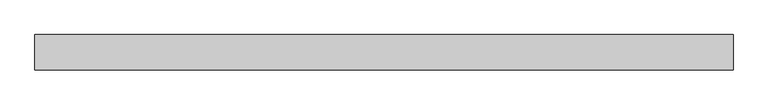
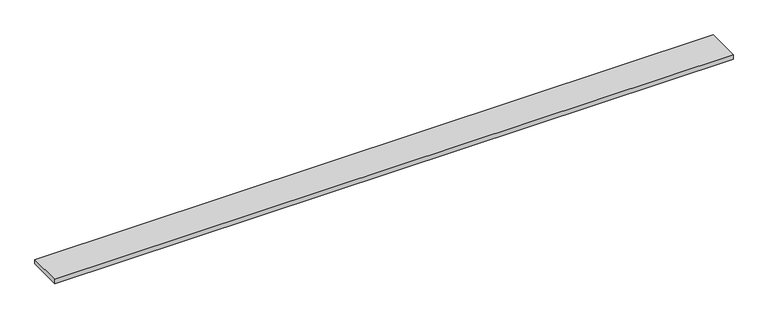
"""IFC4 building model written with IfcOpenShell, lengths in millimetres: proxy geometry, Generic Models 7:Generic Models 1:337419:Generic Models 1:337419 : Generic Models 7:Generic Models 1:337419:27 : Generic Models 7:Generic Models 1:337419:Generic Models 1:337419 : Generic Models 7:Generic Models 1:337419:301336."""

from ifc_helpers import new_model, si_unit, frame, origin, place, context, project, spatial, polyline, outline, extrude, source, transform, mapped, element, save


def generic_models_7370aaea(model_context):
    return source(origin(), model_context, "Body", "SweptSolid", [
        extrude(outline(polyline([(596182.8367242, -567935.4195091), (596182.8367242, -568183.8632591), (591306.0367242, -568183.8632591), (591306.0367242, -567935.4195091), (596182.8367242, -567935.4195091)])), frame((0.0, 0.0, 2489.1643609), z_axis=(0.0, 0.0, 1.0), x_axis=(1.0, 0.0, 0.0)), (0.0, 0.0, 1.0), 32.8770453),
    ])


if __name__ == "__main__":
    model = new_model("IFC4")
    model_context = context("Model", 3, world=origin())
    ifc_project = project(units=[si_unit("LENGTHUNIT", "METRE", prefix="MILLI")], contexts=[model_context])
    site = spatial("IfcSite", under=ifc_project)
    building = spatial("IfcBuilding", under=site)
    placement = place(None, origin())
    generic_models_shape = generic_models_7370aaea(model_context)
    element("IfcBuildingElementProxy", 1, Name="Generic Models 7:Generic Models 1:337419:Generic Models 1:337419 : Generic Models 7:Generic Models 1:337419:27 : Generic Models 7:Generic Models 1:337419:Generic Models 1:337419 : Generic Models 7:Generic Models 1:337419:301336", ObjectType="Generic Models 7:Generic Models 1:337419:Generic Models 1:337419 : Generic Models 7:Generic Models 1:337419:27 : Generic Models 7:Generic Models 1:337419:Generic Models 1:337419 : Generic Models 7:Generic Models 1:337419:301336", at=placement, inside=building, context=model_context, shape_type="MappedRepresentation", body=[
        mapped(generic_models_shape, transform((0.0, 0.0, 0.0), x_axis=(1.0, 0.0, 0.0), y_axis=(0.0, 1.0, 0.0), z_axis=(0.0, 0.0, 1.0))),
    ])
    save(model, "model.ifc")

# Revit data of these elements
# Type "Generic Models 7:Generic Models 1:337419:Generic Models 1:337419 : Generic Models 7:Generic Models 1:337419:27 : Generic Models 7:Generic Models 1:337419:Generic Models 1:337419 : Generic Models 7:Generic Models 1:337419:301336"
#   NameOverride = "Generic Models 7:Generic Models 1:337419:Generic Models 1:337419 : Generic Models 7:Generic Models 1:337419:301336"
#   ObjectTypeOverride = "Generic Models 1:337419 : Generic Models 7:Generic Models 1:337419"
#   Reference = "Generic Models 1"
#   Tag = "301336"
# Element 1 (IfcBuildingElementProxy, "Generic Models 7:Generic Models 1:337419:Generic Models 1:337419 : Generic Models 7:Generic Models 1:337419:27 : Generic Models 7:Generic Models 1:337419:Generic Models 1:337419 : Generic Models 7:Generic Models 1:337419:301336")
#   Materials on its faces: "BLOCKING - SIZE AS NEC."
# Materials
#   "BLOCKING - SIZE AS NEC.": class "Wood", colour RGB 144 113 62, transparency 0, Description = "Pinus Echinata", Cost = 0
